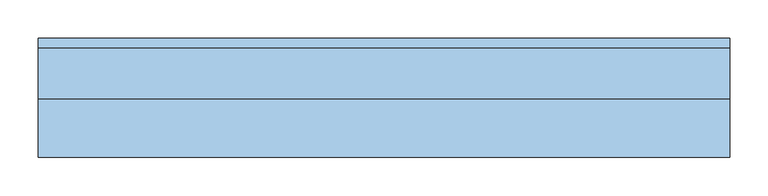
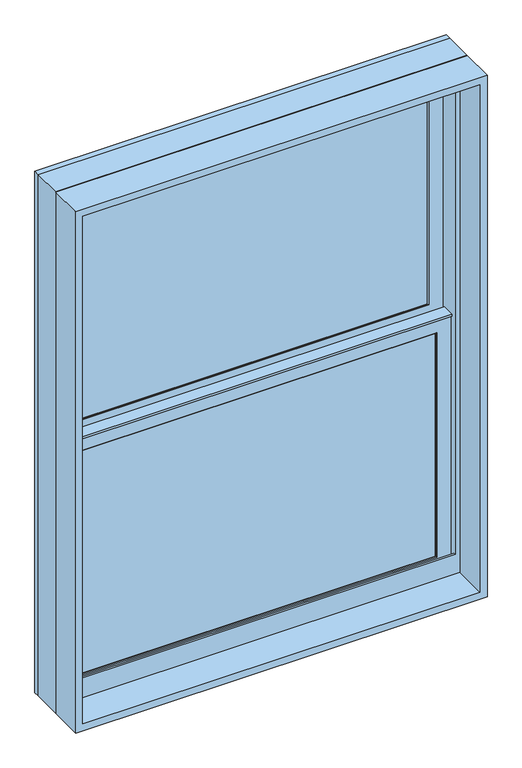
"""IFC4 building model written with IfcOpenShell, lengths in millimetres: window geometry, Window-Double_Hung-Marvin-Essential : ESDH3040."""

from ifc_helpers import new_model, si_unit, frame, origin, place, context, project, spatial, polyline, outline, extrude, faceted_brep, source, transform, mapped, element, save


def window_ecfb91aa(model_context):
    return source(origin(), model_context, "Body", "SolidModel", [
        extrude(outline(polyline([(140.7583333, 20.6375), (140.7583333, 15.875), (121.7083333, 15.875), (121.7083333, 20.6375), (140.7583333, 20.6375)])), frame((0.0, 0.0, 1289.05), z_axis=(0.0, 0.0, 1.0), x_axis=(1.0, 0.0, 0.0)), (0.0, 0.0, 1.0), 527.05),
        extrude(outline(polyline([(-121.7083333, 20.6375), (-121.7083333, 15.875), (-140.7583333, 15.875), (-140.7583333, 20.6375), (-121.7083333, 20.6375)])), frame((0.0, 0.0, 1289.05), z_axis=(0.0, 0.0, 1.0), x_axis=(1.0, 0.0, 0.0)), (0.0, 0.0, 1.0), 527.05),
        extrude(outline(polyline([(393.7, 20.6375), (393.7, 15.875), (-393.7, 15.875), (-393.7, 20.6375), (393.7, 20.6375)])), frame((0.0, 0.0, 1543.05), z_axis=(0.0, 0.0, 1.0), x_axis=(1.0, 0.0, 0.0)), (0.0, 0.0, 1.0), 19.05),
        extrude(outline(polyline([(-140.7583333, 46.83125), (-140.7583333, 51.59375), (-121.7083333, 51.59375), (-121.7083333, 46.83125), (-140.7583333, 46.83125)])), frame((0.0, 0.0, 1854.2), z_axis=(0.0, 0.0, 1.0), x_axis=(1.0, 0.0, 0.0)), (0.0, 0.0, 1.0), 527.05),
        extrude(outline(polyline([(121.7083333, 46.83125), (121.7083333, 51.59375), (140.7583333, 51.59375), (140.7583333, 46.83125), (121.7083333, 46.83125)])), frame((0.0, 0.0, 1854.2), z_axis=(0.0, 0.0, 1.0), x_axis=(1.0, 0.0, 0.0)), (0.0, 0.0, 1.0), 527.05),
        extrude(outline(polyline([(-393.7, 46.83125), (-393.7, 51.59375), (393.7, 51.59375), (393.7, 46.83125), (-393.7, 46.83125)])), frame((0.0, 0.0, 2108.2), z_axis=(0.0, 0.0, 1.0), x_axis=(1.0, 0.0, 0.0)), (0.0, 0.0, 1.0), 19.05),
        extrude(outline(polyline([(140.7583333, 20.6375), (121.7083333, 20.6375), (121.7083333, 25.4), (140.7583333, 25.4), (140.7583333, 20.6375)])), frame((0.0, 0.0, 1289.05), z_axis=(0.0, 0.0, 1.0), x_axis=(1.0, 0.0, 0.0)), (0.0, 0.0, 1.0), 527.05),
        extrude(outline(polyline([(-121.7083333, 20.6375), (-140.7583333, 20.6375), (-140.7583333, 25.4), (-121.7083333, 25.4), (-121.7083333, 20.6375)])), frame((0.0, 0.0, 1289.05), z_axis=(0.0, 0.0, 1.0), x_axis=(1.0, 0.0, 0.0)), (0.0, 0.0, 1.0), 527.05),
        extrude(outline(polyline([(393.7, 20.6375), (-393.7, 20.6375), (-393.7, 25.4), (393.7, 25.4), (393.7, 20.6375)])), frame((0.0, 0.0, 1543.05), z_axis=(0.0, 0.0, 1.0), x_axis=(1.0, 0.0, 0.0)), (0.0, 0.0, 1.0), 19.05),
        extrude(outline(polyline([(-140.7583333, 56.35625), (-121.7083333, 56.35625), (-121.7083333, 51.59375), (-140.7583333, 51.59375), (-140.7583333, 56.35625)])), frame((0.0, 0.0, 1854.2), z_axis=(0.0, 0.0, 1.0), x_axis=(1.0, 0.0, 0.0)), (0.0, 0.0, 1.0), 527.05),
        extrude(outline(polyline([(121.7083333, 56.35625), (140.7583333, 56.35625), (140.7583333, 51.59375), (121.7083333, 51.59375), (121.7083333, 56.35625)])), frame((0.0, 0.0, 1854.2), z_axis=(0.0, 0.0, 1.0), x_axis=(1.0, 0.0, 0.0)), (0.0, 0.0, 1.0), 527.05),
        extrude(outline(polyline([(-393.7, 56.35625), (393.7, 56.35625), (393.7, 51.59375), (-393.7, 51.59375), (-393.7, 56.35625)])), frame((0.0, 0.0, 2108.2), z_axis=(0.0, 0.0, 1.0), x_axis=(1.0, 0.0, 0.0)), (0.0, 0.0, 1.0), 19.05),
        faceted_brep([(-420.6875, 5.6780605, 1846.1351748), (-420.6875, 5.6780605, 1841.5), (420.6875, 5.6780605, 1841.5), (420.6875, 5.6780605, 1846.1351748), (-420.6875, 34.8118605, 1846.1351748), (420.6875, 34.8118605, 1846.1351748), (420.6875, 34.8118605, 1841.5), (-420.6875, 34.8118605, 1841.5), (-420.6875, 30.1625, 1841.5), (-420.6875, 30.1625, 1262.0625), (-420.6875, 8.9241104, 1262.0625), (-420.6875, 8.9241104, 1841.5), (420.6875, 8.9241104, 1841.5), (420.6875, 30.1625, 1841.5), (420.6875, 8.9241104, 1262.0625), (420.6875, 30.1625, 1262.0625), (-404.8034752, 11.90625, 1827.2034752), (-404.8034752, 30.1625, 1827.2034752), (404.8034752, 30.1625, 1827.2034752), (404.8034752, 11.90625, 1827.2034752), (-388.14375, 10.4662439, 1810.54375), (-388.14375, 11.90625, 1810.54375), (388.14375, 11.90625, 1810.54375), (388.14375, 10.4662439, 1810.54375), (389.6858834, 8.9241104, 1812.0858834), (-389.6858834, 8.9241104, 1812.0858834), (404.8034752, 30.1625, 1277.9465248), (404.8034752, 11.90625, 1277.9465248), (388.14375, 11.90625, 1294.60625), (388.14375, 10.4662439, 1294.60625), (389.6858834, 8.9241104, 1293.0641166), (-404.8034752, 30.1625, 1277.9465248), (-404.8034752, 11.90625, 1277.9465248), (-388.14375, 11.90625, 1294.60625), (-388.14375, 10.4662439, 1294.60625), (-389.6858834, 8.9241104, 1293.0641166)], [[[0, 1, 2, 3]], [[4, 5, 6, 7]], [[1, 0, 4, 7, 8, 9, 10, 11]], [[2, 1, 11, 12]], [[7, 6, 13, 8]], [[3, 2, 12, 14, 15, 13, 6, 5]], [[0, 3, 5, 4]], [[16, 17, 18, 19]], [[20, 21, 22, 23]], [[20, 23, 24, 25]], [[19, 18, 26, 27]], [[23, 22, 28, 29]], [[24, 23, 29, 30]], [[27, 26, 31, 32]], [[29, 28, 33, 34]], [[30, 29, 34, 35]], [[15, 14, 10, 9]], [[15, 9, 8, 13], [18, 17, 31, 26]], [[17, 16, 32, 31]], [[16, 19, 27, 32], [22, 21, 33, 28]], [[21, 20, 34, 33]], [[20, 25, 35, 34]], [[10, 14, 12, 11], [25, 24, 30, 35]]]),
        extrude(outline(polyline([(38.5955581, 1827.2125), (33.5778968, 1827.2125), (33.5778968, 1828.8), (39.9405976, 1828.8), (39.9405976, 1827.2125), (61.515625, 1827.2125), (47.6307501, 1823.8975159), (38.5955581, 1823.8975159), (38.5955581, 1827.2125)])), frame((-420.6875, 0.0, 0.0), z_axis=(1.0, 0.0, 0.0), x_axis=(0.0, 1.0, 0.0)), (0.0, 0.0, 1.0), 841.375),
        faceted_brep([(450.85, 0.0, 1231.9), (450.85, 0.0, 2438.4), (-450.85, 0.0, 2438.4), (-450.85, 0.0, 1231.9), (424.65625, 0.0, 1293.01875), (-424.65625, 0.0, 1293.01875), (-424.65625, 0.0, 2412.20625), (424.65625, 0.0, 2412.20625), (424.65625, 3.96875, 1231.9), (-424.65625, 3.96875, 1231.9), (-424.65625, 3.96875, 1293.01875), (424.65625, 3.96875, 1293.01875), (-450.85, 65.6828125, 1231.9), (-424.65625, 65.6828125, 1231.9), (424.65625, 65.6828125, 1231.9), (450.85, 65.6828125, 1231.9), (-450.85, 65.6828125, 2438.4), (450.85, 65.6828125, 2438.4), (424.65625, 65.6828125, 2412.20625), (-424.65625, 65.6828125, 2412.20625)], [[[0, 1, 2, 3], [4, 5, 6, 7]], [[8, 9, 10, 11]], [[5, 4, 11, 10]], [[0, 3, 12, 13, 9, 8, 14, 15]], [[13, 12, 16, 17, 15, 14, 18, 19]], [[13, 19, 6, 5, 10, 9]], [[7, 6, 19, 18]], [[18, 14, 8, 11, 4, 7]], [[1, 0, 15, 17]], [[2, 1, 17, 16]], [[3, 2, 16, 12]]]),
        faceted_brep([(424.65625, 30.1625, 1835.15), (423.06875, 30.1625, 1835.15), (423.06875, 30.1625, 1256.2544613), (424.65625, 30.1625, 1256.2544613), (-423.06875, 30.1625, 1835.15), (-424.65625, 30.1625, 1835.15), (-424.65625, 30.1625, 1256.2544613), (-423.06875, 30.1625, 1256.2544613), (423.06875, 63.5, 1835.15), (424.65625, 63.5, 1835.15), (424.65625, 63.5, 1249.7743077), (423.06875, 63.5, 1249.7743077), (-424.65625, 63.5, 1835.15), (-423.06875, 63.5, 1835.15), (-423.06875, 63.5, 1249.7743077), (-424.65625, 63.5, 1249.7743077), (435.9108932, 3.96875, 1261.3460105), (435.9108932, 3.96875, 1231.9), (435.9108932, 65.6828125, 1231.9), (435.9108932, 65.6828125, 1249.350012), (-435.9108932, 3.96875, 1231.9), (-435.9108932, 3.96875, 1261.3460105), (-435.9108932, 65.6828125, 1249.350012), (-435.9108932, 65.6828125, 1231.9), (435.9108932, 78.58125, 1246.8428097), (-435.9108932, 78.58125, 1246.8428097), (-433.8971252, 68.2348864, 1248.8539391), (-415.93135, 68.2348864, 1248.8539391), (-415.93135, 65.6828125, 1249.350012), (415.93135, 65.6828125, 1249.350012), (415.93135, 68.2348864, 1248.8539391), (433.8971252, 68.2348864, 1248.8539391), (-450.85, 65.6828125, 1231.9), (-450.85, 78.5948249, 1231.9), (450.85, 78.5948249, 1231.9), (450.85, 65.6828125, 1231.9), (-450.85, 78.58125, 2438.4), (450.85, 78.58125, 2438.4), (435.9108932, 78.58125, 2423.4608932), (-435.9108932, 78.58125, 2423.4608932), (-450.85, 65.6828125, 2438.4), (-433.8971252, 68.2348864, 2421.4471252), (433.8971252, 68.2348864, 2421.4471252), (415.93135, 68.2348864, 2403.48135), (-415.93135, 68.2348864, 2403.48135), (-415.93135, 65.6828125, 2403.48135), (415.93135, 65.6828125, 2403.48135), (450.85, 65.6828125, 2438.4)], [[[0, 1, 2, 3]], [[4, 5, 6, 7]], [[8, 9, 10, 11]], [[12, 13, 14, 15]], [[1, 8, 11, 2]], [[9, 0, 3, 10]], [[1, 0, 9, 8]], [[5, 4, 13, 12]], [[5, 12, 15, 6]], [[13, 4, 7, 14]], [[16, 17, 18, 19]], [[20, 21, 22, 23]], [[24, 25, 26, 27, 28, 22, 21, 16, 19, 29, 30, 31], [3, 2, 11, 10], [7, 6, 15, 14]], [[17, 16, 21, 20]], [[17, 20, 23, 32, 33, 34, 35, 18]], [[34, 33, 36, 37], [25, 24, 38, 39]], [[33, 32, 40, 36]], [[39, 41, 26, 25]], [[41, 42, 31, 30, 43, 44, 27, 26]], [[44, 45, 28, 27]], [[40, 32, 23, 22, 28, 45, 46, 29, 19, 18, 35, 47]], [[36, 40, 47, 37]], [[39, 38, 42, 41]], [[44, 43, 46, 45]], [[34, 37, 47, 35]], [[42, 38, 24, 31]], [[46, 43, 30, 29]]]),
        extrude(outline(polyline([(400.84375, 11.90625), (-400.84375, 11.90625), (-400.84375, 15.08125), (400.84375, 15.08125), (400.84375, 11.90625)])), frame((0.0, 0.0, 1281.90625), z_axis=(0.0, 0.0, 1.0), x_axis=(1.0, 0.0, 0.0)), (0.0, 0.0, 1.0), 541.3375),
        extrude(outline(polyline([(400.84375, 42.8625), (-400.84375, 42.8625), (-400.84375, 46.0375), (400.84375, 46.0375), (400.84375, 42.8625)])), frame((0.0, 0.0, 1847.05625), z_axis=(0.0, 0.0, 1.0), x_axis=(1.0, 0.0, 0.0)), (0.0, 0.0, 1.0), 541.3375),
        faceted_brep([(-388.14375, 31.194477, 1810.54375), (-389.6858834, 32.7366104, 1812.0858834), (389.6858834, 32.7366104, 1812.0858834), (388.14375, 31.194477, 1810.54375), (-388.14375, 30.1625, 1810.54375), (388.14375, 30.1625, 1810.54375), (-420.6875, 32.7366104, 1843.0875), (-420.6875, 30.1625, 1843.0875), (420.6875, 30.1625, 1843.0875), (420.6875, 32.7366104, 1843.0875), (389.6858834, 32.7366104, 1293.0641166), (388.14375, 31.194477, 1294.60625), (388.14375, 30.1625, 1294.60625), (420.6875, 30.1625, 1262.0625), (420.6875, 32.7366104, 1262.0625), (-389.6858834, 32.7366104, 1293.0641166), (-388.14375, 31.194477, 1294.60625), (-388.14375, 30.1625, 1294.60625), (-420.6875, 30.1625, 1262.0625), (-420.6875, 32.7366104, 1262.0625)], [[[0, 1, 2, 3]], [[4, 0, 3, 5]], [[6, 7, 8, 9]], [[3, 2, 10, 11]], [[5, 3, 11, 12]], [[9, 8, 13, 14]], [[11, 10, 15, 16]], [[12, 11, 16, 17]], [[14, 13, 18, 19]], [[9, 14, 19, 6], [1, 15, 10, 2]], [[16, 15, 1, 0]], [[17, 16, 0, 4]], [[7, 18, 13, 8], [5, 12, 17, 4]], [[19, 18, 7, 6]]]),
        faceted_brep([(-404.8034752, 42.8625, 2392.3534752), (-404.8034752, 61.11875, 2392.3534752), (404.8034752, 61.11875, 2392.3534752), (404.8034752, 42.8625, 2392.3534752), (-388.14375, 41.4224939, 2375.69375), (-388.14375, 42.8625, 2375.69375), (388.14375, 42.8625, 2375.69375), (388.14375, 41.4224939, 2375.69375), (-389.6858834, 39.8803604, 2377.2358834), (389.6858834, 39.8803604, 2377.2358834), (-420.6875, 61.11875, 2408.2375), (-420.6875, 39.8803604, 2408.2375), (420.6875, 39.8803604, 2408.2375), (420.6875, 61.11875, 2408.2375), (404.8034752, 61.11875, 1843.0965248), (404.8034752, 42.8625, 1843.0965248), (388.14375, 42.8625, 1859.75625), (388.14375, 41.4224939, 1859.75625), (389.6858834, 39.8803604, 1858.2141166), (420.6875, 39.8803604, 1827.2125), (420.6875, 61.11875, 1827.2125), (-404.8034752, 61.11875, 1843.0965248), (-404.8034752, 42.8625, 1843.0965248), (-388.14375, 42.8625, 1859.75625), (-388.14375, 41.4224939, 1859.75625), (-389.6858834, 39.8803604, 1858.2141166), (-420.6875, 39.8803604, 1827.2125), (-420.6875, 61.11875, 1827.2125)], [[[0, 1, 2, 3]], [[4, 5, 6, 7]], [[8, 4, 7, 9]], [[10, 11, 12, 13]], [[3, 2, 14, 15]], [[7, 6, 16, 17]], [[9, 7, 17, 18]], [[13, 12, 19, 20]], [[15, 14, 21, 22]], [[17, 16, 23, 24]], [[18, 17, 24, 25]], [[20, 19, 26, 27]], [[13, 20, 27, 10], [1, 21, 14, 2]], [[22, 21, 1, 0]], [[3, 15, 22, 0], [5, 23, 16, 6]], [[24, 23, 5, 4]], [[25, 24, 4, 8]], [[11, 26, 19, 12], [9, 18, 25, 8]], [[27, 26, 11, 10]]]),
        faceted_brep([(-420.6875, 61.11875, 1827.2125), (-420.6875, 63.6928604, 1827.2125), (420.6875, 63.6928604, 1827.2125), (420.6875, 61.11875, 1827.2125), (-388.14375, 62.150727, 1859.75625), (-388.14375, 61.11875, 1859.75625), (388.14375, 61.11875, 1859.75625), (388.14375, 62.150727, 1859.75625), (-389.6858834, 63.6928604, 1858.2141166), (389.6858834, 63.6928604, 1858.2141166), (420.6875, 63.6928604, 2408.2375), (420.6875, 61.11875, 2408.2375), (388.14375, 61.11875, 2375.69375), (388.14375, 62.150727, 2375.69375), (389.6858834, 63.6928604, 2377.2358834), (-420.6875, 63.6928604, 2408.2375), (-420.6875, 61.11875, 2408.2375), (-388.14375, 61.11875, 2375.69375), (-388.14375, 62.150727, 2375.69375), (-389.6858834, 63.6928604, 2377.2358834)], [[[0, 1, 2, 3]], [[4, 5, 6, 7]], [[8, 4, 7, 9]], [[3, 2, 10, 11]], [[7, 6, 12, 13]], [[9, 7, 13, 14]], [[11, 10, 15, 16]], [[13, 12, 17, 18]], [[14, 13, 18, 19]], [[16, 15, 1, 0]], [[3, 11, 16, 0], [5, 17, 12, 6]], [[18, 17, 5, 4]], [[19, 18, 4, 8]], [[1, 15, 10, 2], [9, 14, 19, 8]]]),
        extrude(outline(polyline([(400.84375, 26.19375), (-400.84375, 26.19375), (-400.84375, 30.1625), (400.84375, 30.1625), (400.84375, 26.19375)])), frame((0.0, 0.0, 1281.90625), z_axis=(0.0, 0.0, 1.0), x_axis=(1.0, 0.0, 0.0)), (0.0, 0.0, 1.0), 541.3375),
        extrude(outline(polyline([(400.84375, 57.15), (-400.84375, 57.15), (-400.84375, 61.11875), (400.84375, 61.11875), (400.84375, 57.15)])), frame((0.0, 0.0, 1847.05625), z_axis=(0.0, 0.0, 1.0), x_axis=(1.0, 0.0, 0.0)), (0.0, 0.0, 1.0), 541.3375),
        extrude(outline(polyline([(2438.4, 450.85), (2438.4, -450.85), (1231.9, -450.85), (1231.9, 450.85), (2438.4, 450.85)]), holes=[polyline([(2422.525, 434.975), (1247.775, 434.975), (1247.775, -434.975), (2422.525, -434.975), (2422.525, 434.975)])]), frame((0.0, -76.2, 0.0), z_axis=(0.0, 1.0, 0.0), x_axis=(0.0, 0.0, 1.0)), (0.0, 0.0, 1.0), 75.40625),
    ])


if __name__ == "__main__":
    model = new_model("IFC4")
    model_context = context("Model", 3, world=origin())
    ifc_project = project(units=[si_unit("LENGTHUNIT", "METRE", prefix="MILLI")], contexts=[model_context])
    site = spatial("IfcSite", under=ifc_project)
    building = spatial("IfcBuilding", under=site)
    placement = place(None, origin())
    window_shape = window_ecfb91aa(model_context)
    element("IfcWindow", 1, ObjectType="Window-Double_Hung-Marvin-Essential : ESDH3040", at=placement, inside=building, context=model_context, shape_type="MappedRepresentation", body=[
        mapped(window_shape, transform((0.0, 0.0, 0.0), x_axis=(1.0, 0.0, 0.0), y_axis=(0.0, 1.0, 0.0), z_axis=(0.0, 0.0, 1.0))),
    ])
    save(model, "model.ifc")

# Revit data of these elements
# Type "Window-Double_Hung-Marvin-Essential : ESDH3040"
#   Type Mark = "51"
#   Window Type = "Essential Double Hung"
#   Product data url = "https://bimobject.com/marvin-windows-and-doors/product/marvin-dhwau"
#   Product Guid = "c4a96547-874c-4385-91dc-a058adc19d98"
#   Frame = "All Ultrex"
#   Egress Window = "No"
#   URL = "www.marvin.com"
#   Model = "ESDH3040"
#   Manufacturer = "Marvin Windows and Doors"
#   Label Egress = ""
#   Glass Type = "IG Low E II with Argon"
#   Design Pressure = "DP50"
#   Description = "3648 DBHG"
#   Analytic Construction = "<None>"
#   Prairie Corner Width = 0' - 4"
#   Prairie Corner Height = 0' - 4"
#   Egress Width = 2' - 8 9/16"
#   Egress Height = 1' - 7 27/128"
#   Rough Width = 3' - 0"
#   Rough Height = 4' - 0"
#   Nominal Width = 3' - 0"
#   Nominal Height = 4' - 0"
#   Inset to Installation Flange [instance default] = 0' - 1"
#   Height = 3' - 11 1/2"
#   Egress Area = 4.34414 SF
#   Default Head Height = 8' - 0"
#   Width = 2' - 11 1/2"
#   Daylight Area = 8.62223 SF
#   DLO Width = 2' - 6 9/16"
#   DLO Height = 1' - 8 5/16"
#   Muntins Top Sash = yes
#   Lites Wide Top Sash = 3
#   Lites Wide Bottom Sash = 3
#   Lites High Top Sash = 2
#   Lites High Bottom Sash = 2
#   Lite Cut Prairie 9 = no
#   Lite Cut HV Grid = yes
#   Muntins Bottom Sash = yes
#   Label Visibility = no
#   Jamb Extension Visibility = yes
#   Edition number = 1
#   Interior Material = Ultrex-Marvin-Stonewhite
#   Glazing Material = Glass-Marvin-IG Low E II with Argon
#   Cladding Material = Ultrex-Marvin-Pebblegray
#   Wall Closure = (empty or 0)
#   Assembly Code = ""
# Element 1 (IfcWindow, "Window-Double_Hung-Marvin-Essential : ESDH3040")
#   Materials on its faces: "Ultrex-Marvin-Pebblegray", "Ultrex-Marvin-Stonewhite", "Glass-Marvin-IG Low E II with Argon"
# Materials
#   "Ultrex-Marvin-Stonewhite": class "Paint", colour RGB 250 251 245, transparency 0
#   "Glass-Marvin-IG Low E II with Argon": class "Glass", colour RGB 0 128 192, transparency 0.85
#   "Ultrex-Marvin-Pebblegray": class "Paint", colour RGB 189 185 173, transparency 0
